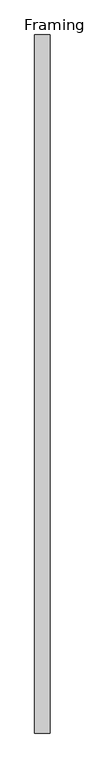
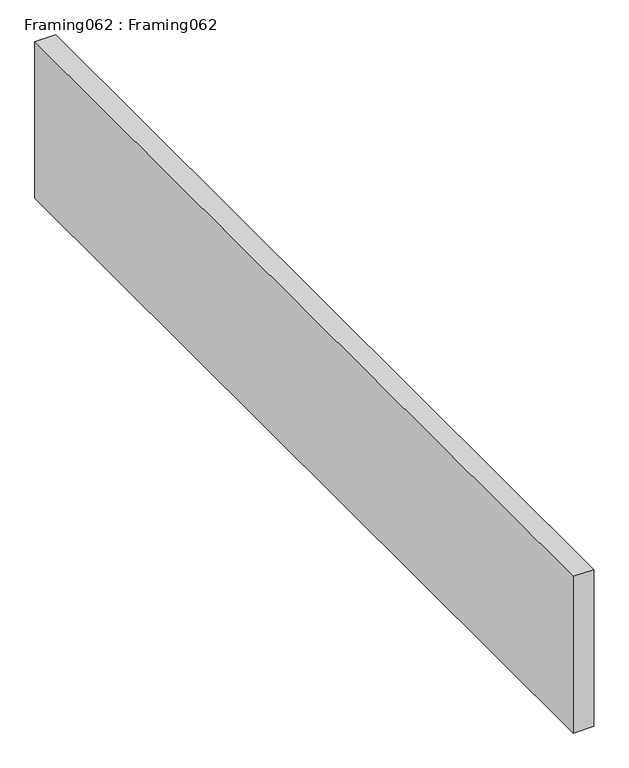
"""IFC4 building model written with IfcOpenShell, lengths in millimetres: proxy geometry, Framing062 : Framing062."""

from ifc_helpers import new_model, si_unit, frame, origin, place, context, project, spatial, polyline, outline, extrude, source, transform, mapped, element, save


def framing062_framing062_1995d564(model_context):
    return source(origin(), model_context, "Body", "SweptSolid", [
        extrude(outline(polyline([(-939.5885697, -1052.8906574), (-984.0385697, -1052.8906574), (-984.0385697, 947.1093426), (-939.5885697, 947.1093426), (-939.5885697, -1052.8906574)])), frame((0.0, 0.0, 42134.105552), z_axis=(0.0, 0.0, 1.0), x_axis=(1.0, 0.0, 0.0)), (0.0, 0.0, 1.0), 355.2981173),
    ])


if __name__ == "__main__":
    model = new_model("IFC4")
    model_context = context("Model", 3, world=origin())
    ifc_project = project(units=[si_unit("LENGTHUNIT", "METRE", prefix="MILLI")], contexts=[model_context])
    site = spatial("IfcSite", under=ifc_project)
    building = spatial("IfcBuilding", under=site)
    placement = place(None, origin())
    framing062_framing062_shape = framing062_framing062_1995d564(model_context)
    element("IfcBuildingElementProxy", 1, Name="Framing062 : Framing062", ObjectType="Framing062 : Framing062", at=placement, inside=building, context=model_context, shape_type="MappedRepresentation", body=[
        mapped(framing062_framing062_shape, transform((0.0, 0.0, 0.0), x_axis=(1.0, 0.0, 0.0), y_axis=(0.0, 1.0, 0.0), z_axis=(0.0, 0.0, 1.0))),
    ])
    save(model, "model.ifc")

# Revit data of these elements
# Type "Framing062 : Framing062"
#   NameOverride = "Framing062"
# Element 1 (IfcBuildingElementProxy, "Framing062 : Framing062")
#   Materials on its faces: "WOOD FRAMING (SEE STRUCT DWGS)"
# Materials
#   "WOOD FRAMING (SEE STRUCT DWGS)": class "Unassigned", colour RGB 224 188 168, transparency 0, Cost = 0
